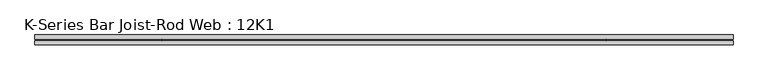
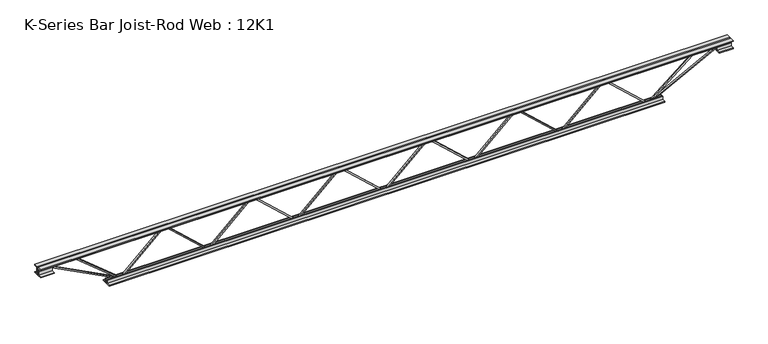
"""IFC4 building model written with IfcOpenShell, lengths in millimetres: beam geometry, K-Series Bar Joist-Rod Web : 12K1."""

from ifc_helpers import new_model, si_unit, frame, origin, place, context, project, spatial, polyline, outline, extrude, source, transform, mapped, element, save


def k_series_bar_joist_rod_web_12k1_c9ffb345(model_context):
    return source(origin(), model_context, "Body", "SweptSolid", [
        extrude(outline(polyline([(-141.2875, 651.9333333), (-150.8125, 651.9333333), (-150.8125, 656.9567529), (141.2875, 976.5734196), (141.2875, 979.2265804), (-150.8125, 1298.8432471), (-150.8125, 1303.8666667), (-141.2875, 1303.8666667), (-141.2875, 1302.5400863), (150.8125, 982.9234196), (150.8125, 972.8765804), (-141.2875, 653.2599137), (-141.2875, 651.9333333)])), frame((0.0, -4.7625, 0.0), z_axis=(0.0, 1.0, 0.0), x_axis=(0.0, 0.0, 1.0)), (0.0, 0.0, 1.0), 9.525),
        extrude(outline(polyline([(-141.2875, 0.0), (-150.8125, 0.0), (-150.8125, 5.0234196), (141.2875, 324.6400863), (141.2875, 327.2932471), (-150.8125, 646.9099137), (-150.8125, 651.9333333), (-141.2875, 651.9333333), (-141.2875, 650.6067529), (150.8125, 330.9900863), (150.8125, 320.9432471), (-141.2875, 1.3265804), (-141.2875, 0.0)])), frame((0.0, -4.7625, 0.0), z_axis=(0.0, 1.0, 0.0), x_axis=(0.0, 0.0, 1.0)), (0.0, 0.0, 1.0), 9.525),
        extrude(outline(polyline([(-141.2875, -651.9333333), (-150.8125, -651.9333333), (-150.8125, -646.9099137), (141.2875, -327.2932471), (141.2875, -324.6400863), (-150.8125, -5.0234196), (-150.8125, 0.0), (-141.2875, 0.0), (-141.2875, -1.3265804), (150.8125, -320.9432471), (150.8125, -330.9900863), (-141.2875, -650.6067529), (-141.2875, -651.9333333)])), frame((0.0, -4.7625, 0.0), z_axis=(0.0, 1.0, 0.0), x_axis=(0.0, 0.0, 1.0)), (0.0, 0.0, 1.0), 9.525),
        extrude(outline(polyline([(-141.2875, -1303.8666667), (-150.8125, -1303.8666667), (-150.8125, -1298.8432471), (141.2875, -979.2265804), (141.2875, -976.5734196), (-150.8125, -656.9567529), (-150.8125, -651.9333333), (-141.2875, -651.9333333), (-141.2875, -653.2599137), (150.8125, -972.8765804), (150.8125, -982.9234196), (-141.2875, -1302.5400863), (-141.2875, -1303.8666667)])), frame((0.0, -4.7625, 0.0), z_axis=(0.0, 1.0, 0.0), x_axis=(0.0, 0.0, 1.0)), (0.0, 0.0, 1.0), 9.525),
        extrude(outline(polyline([(-141.2875, 1303.8666667), (-150.8125, 1303.8666667), (-150.8125, 1308.8900863), (141.2875, 1628.5067529), (141.2875, 1631.1599137), (-150.8125, 1950.7765804), (-150.8125, 1955.8), (-141.2875, 1955.8), (-141.2875, 1954.4734196), (150.8125, 1634.8567529), (150.8125, 1624.8099137), (-141.2875, 1305.1932471), (-141.2875, 1303.8666667)])), frame((0.0, -4.7625, 0.0), z_axis=(0.0, 1.0, 0.0), x_axis=(0.0, 0.0, 1.0)), (0.0, 0.0, 1.0), 9.525),
        extrude(outline(polyline([(-141.2875, -1955.8), (-150.8125, -1955.8), (-150.8125, -1950.7765804), (141.2875, -1631.1599137), (141.2875, -1628.5067529), (-150.8125, -1308.8900863), (-150.8125, -1303.8666667), (-141.2875, -1303.8666667), (-141.2875, -1305.1932471), (150.8125, -1624.8099137), (150.8125, -1634.8567529), (-141.2875, -1954.4734196), (-141.2875, -1955.8)])), frame((0.0, -4.7625, 0.0), z_axis=(0.0, 1.0, 0.0), x_axis=(0.0, 0.0, 1.0)), (0.0, 0.0, 1.0), 9.525),
        extrude(outline(polyline([(4.7625, 152.4), (36.5125, 152.4), (36.5125, 146.05), (11.1125, 146.05), (11.1125, 120.65), (4.7625, 120.65), (4.7625, 152.4)])), frame((-2565.4, 0.0, 0.0), z_axis=(1.0, 0.0, 0.0), x_axis=(0.0, 1.0, 0.0)), (0.0, 0.0, 1.0), 5130.8),
        extrude(outline(polyline([(-4.7625, 152.4), (-4.7625, 120.65), (-11.1125, 120.65), (-11.1125, 146.05), (-36.5125, 146.05), (-36.5125, 152.4), (-4.7625, 152.4)])), frame((-2565.4, 0.0, 0.0), z_axis=(1.0, 0.0, 0.0), x_axis=(0.0, 1.0, 0.0)), (0.0, 0.0, 1.0), 5130.8),
        extrude(outline(polyline([(-4.7625, 88.9), (-36.5125, 88.9), (-36.5125, 95.25), (-11.1125, 95.25), (-11.1125, 120.65), (-4.7625, 120.65), (-4.7625, 88.9)])), frame((-2565.4, 0.0, 0.0), z_axis=(1.0, 0.0, 0.0), x_axis=(0.0, 1.0, 0.0)), (0.0, 0.0, 1.0), 101.6),
        extrude(outline(polyline([(36.5125, 88.9), (4.7625, 88.9), (4.7625, 120.65), (11.1125, 120.65), (11.1125, 95.25), (36.5125, 95.25), (36.5125, 88.9)])), frame((-2565.4, 0.0, 0.0), z_axis=(1.0, 0.0, 0.0), x_axis=(0.0, 1.0, 0.0)), (0.0, 0.0, 1.0), 101.6),
        extrude(outline(polyline([(4.7625, 88.9), (4.7625, 120.65), (11.1125, 120.65), (11.1125, 95.25), (36.5125, 95.25), (36.5125, 88.9), (4.7625, 88.9)])), frame((2463.8, 0.0, 0.0), z_axis=(1.0, 0.0, 0.0), x_axis=(0.0, 1.0, 0.0)), (0.0, 0.0, 1.0), 101.6),
        extrude(outline(polyline([(-4.7625, 88.9), (-36.5125, 88.9), (-36.5125, 95.25), (-11.1125, 95.25), (-11.1125, 120.65), (-4.7625, 120.65), (-4.7625, 88.9)])), frame((2463.8, 0.0, 0.0), z_axis=(1.0, 0.0, 0.0), x_axis=(0.0, 1.0, 0.0)), (0.0, 0.0, 1.0), 101.6),
        extrude(outline(polyline([(4.7625, -152.4), (4.7625, -120.65), (11.1125, -120.65), (11.1125, -146.05), (36.5125, -146.05), (36.5125, -152.4), (4.7625, -152.4)])), frame((-2057.4, 0.0, 0.0), z_axis=(1.0, 0.0, 0.0), x_axis=(0.0, 1.0, 0.0)), (0.0, 0.0, 1.0), 4114.8),
        extrude(outline(polyline([(-4.7625, -152.4), (-36.5125, -152.4), (-36.5125, -146.05), (-11.1125, -146.05), (-11.1125, -120.65), (-4.7625, -120.65), (-4.7625, -152.4)])), frame((-2057.4, 0.0, 0.0), z_axis=(1.0, 0.0, 0.0), x_axis=(0.0, 1.0, 0.0)), (0.0, 0.0, 1.0), 4114.8),
        extrude(outline(polyline([(0.0, -9.525), (0.0, 0.0), (573.7533355, 0.0), (573.7533355, -9.525), (0.0, -9.525)])), frame((-2466.0137714, 4.7625, 116.4332925), z_axis=(0.464833898989514, 0.0, 0.8853979028381569), x_axis=(0.8853979028381569, 0.0, -0.464833898989514)), (0.0, 0.0, 1.0), 9.525),
        extrude(outline(polyline([(0.0, -9.525), (0.0, 0.0), (421.1687996, 0.0), (421.1687996, -9.525), (0.0, -9.525)])), frame((-2284.7824616, 4.7625, 116.9640284), z_axis=(0.633237790256868, 0.0, 0.773957299203644), x_axis=(0.773957299203644, 0.0, -0.633237790256868)), (0.0, 0.0, 1.0), 9.525),
        extrude(outline(polyline([(0.0, -9.525), (0.0, 0.0), (573.7533355, 0.0), (573.7533355, -9.525), (0.0, -9.525)])), frame((2466.0137714, -4.7625, 116.4332925), z_axis=(-0.4648338989894958, 0.0, 0.8853979028381664), x_axis=(-0.8853979028381664, 0.0, -0.4648338989894958)), (0.0, 0.0, 1.0), 9.525),
        extrude(outline(polyline([(0.0, -9.525), (0.0, 0.0), (421.1687996, 0.0), (421.1687996, -9.525), (0.0, -9.525)])), frame((2284.7824616, -4.7625, 116.9640284), z_axis=(-0.6332377902568614, 0.0, 0.7739572992036493), x_axis=(-0.7739572992036493, 0.0, -0.6332377902568614)), (0.0, 0.0, 1.0), 9.525),
    ])


if __name__ == "__main__":
    model = new_model("IFC4")
    model_context = context("Model", 3, world=origin())
    ifc_project = project(units=[si_unit("LENGTHUNIT", "METRE", prefix="MILLI")], contexts=[model_context])
    site = spatial("IfcSite", under=ifc_project)
    building = spatial("IfcBuilding", under=site)
    placement = place(None, origin())
    k_series_bar_joist_rod_web_12k1_shape = k_series_bar_joist_rod_web_12k1_c9ffb345(model_context)
    element("IfcBeam", 1, ObjectType="K-Series Bar Joist-Rod Web : 12K1", at=placement, inside=building, context=model_context, shape_type="MappedRepresentation", body=[
        mapped(k_series_bar_joist_rod_web_12k1_shape, transform((0.0, 0.0, 0.0), x_axis=(1.0, 0.0, 0.0), y_axis=(0.0, 1.0, 0.0), z_axis=(0.0, 0.0, 1.0))),
    ])
    save(model, "model.ifc")

# Revit data of these elements
# Type "K-Series Bar Joist-Rod Web : 12K1"
#   Assembly Code = "B1010350"
#   Wt = 5
#   Web Thickness = 0' - 0 3/8"
#   Start Offset [instance default] = 0' - 0"
#   Start Extension [instance default] = 0' - 0"
#   Seat Length = 0' - 4"
#   Seat Depth = 0' - 2 1/2"
#   PanelArrayLength [instance default] = 20' - 0"
#   Panel [instance default] = 2' - 0"
#   End Offset [instance default] = 0' - 0"
#   End Extension [instance default] = 0' - 0"
#   End Panel = 2' - 0"
#   Cord Leg = 0' - 1 1/4"
#   Chord Thickness = 0' - 0 1/4"
#   Length [instance default] = 24' - 0"
#   Depth = 1' - 0"
#   PanelArrayNum [instance default] = 10
#   Structural Material = none
# Element 1 (IfcBeam, "K-Series Bar Joist-Rod Web : 12K1")
#   PanelArrayLength = 12' - 10"
#   Panel = 2' - 1.66667"
#   PanelArrayNum = 6
